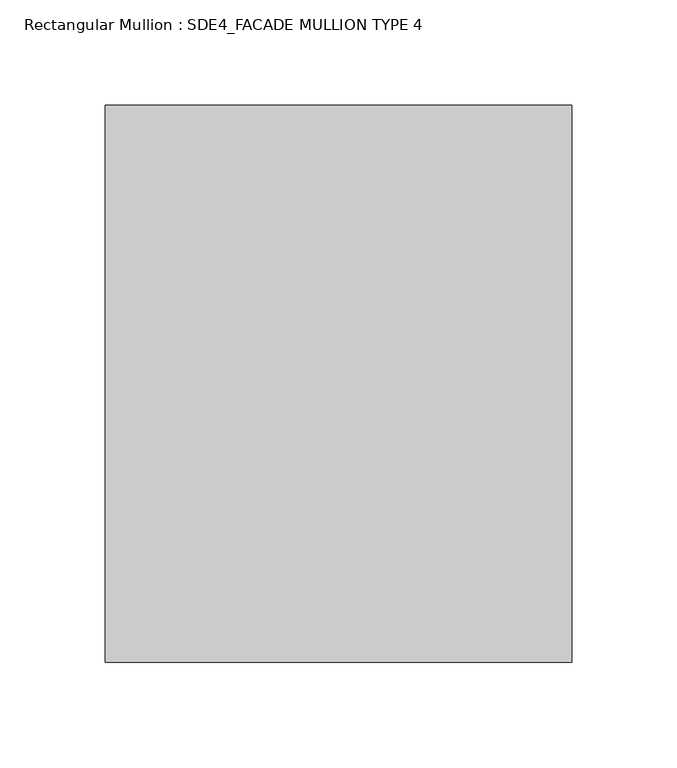
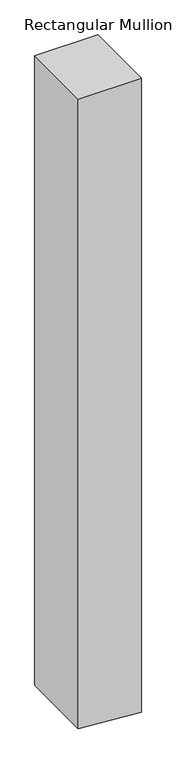
"""IFC4 building model written with IfcOpenShell, lengths in millimetres: member geometry, Rectangular Mullion : SDE4_FACADE MULLION TYPE 4."""

import ifcopenshell
import ifcopenshell.guid

model = None  # the IFC model being written
_history = None  # IfcOwnerHistory: only IFC2X3 demands one
_inside = {}  # id of a spatial element -> (the spatial element, [elements in it])
_under = {}  # id of a project, library or spatial element -> (it, [spatial elements below it])
_declared = {}  # id of a project -> (the project, [libraries it declares])
_typed = {}  # id of a type object -> (the type object, [elements of that type])
_made_of = {}  # id of a material, layer set ... -> (it, [elements and type objects made of it])


def new_model(schema):
    """Start an empty IFC model of exactly this schema.

    Asked for "IFC4X3", IfcOpenShell would pick the latest addendum, in which some entities
    have other attributes; the version numbers below select the first issue.
    IFC2X3 requires an IfcOwnerHistory on every rooted entity: one is made here for all.
    """
    global model, _history
    if schema == "IFC4X3":
        model = ifcopenshell.file(schema_version=(4, 3, 0, 0))
    else:
        model = ifcopenshell.file(schema=schema)
    _inside.clear()
    _under.clear()
    _declared.clear()
    _typed.clear()
    _made_of.clear()
    _history = None
    if model.schema == "IFC2X3":
        org = make("IfcOrganization", Name="unknown")
        user = make(
            "IfcPersonAndOrganization",
            ThePerson=make("IfcPerson", FamilyName="unknown"),
            TheOrganization=org,
        )
        app = make(
            "IfcApplication",
            ApplicationDeveloper=org,
            Version="unknown",
            ApplicationFullName="unknown",
            ApplicationIdentifier="unknown",
        )
        _history = make(
            "IfcOwnerHistory",
            OwningUser=user,
            OwningApplication=app,
            ChangeAction="ADDED",
            CreationDate=0,
        )
    return model


def make(cls, **values):
    """One entity of the class cls with the attributes given. An attribute that is None is left unset."""
    return model.create_entity(
        cls, **{name: value for name, value in values.items() if value is not None}
    )


def rooted(cls, **values):
    """An entity with a GlobalId (a new one), such as an element, a storey or a relation."""
    return make(cls, GlobalId=ifcopenshell.guid.new(), OwnerHistory=_history, **values)


def si_unit(unit_type, name, prefix=None):
    """IfcSIUnit, for example si_unit("LENGTHUNIT", "METRE", prefix="MILLI")."""
    return make("IfcSIUnit", UnitType=unit_type, Prefix=prefix, Name=name)


def assignment(units):
    """IfcUnitAssignment: the units of a project."""
    return None if units is None else make("IfcUnitAssignment", Units=units)


def point(xyz):
    """IfcCartesianPoint."""
    return None if xyz is None else make("IfcCartesianPoint", Coordinates=xyz)


def direction(xyz):
    """IfcDirection."""
    return None if xyz is None else make("IfcDirection", DirectionRatios=xyz)


def frame(location, z_axis=None, x_axis=None):
    """IfcAxis2Placement3D, a coordinate frame: its origin and axes. An axis left out is left unset."""
    return make(
        "IfcAxis2Placement3D",
        Location=point(location),
        Axis=direction(z_axis),
        RefDirection=direction(x_axis),
    )


def origin():
    """The frame at (0, 0, 0) with its axes left unset."""
    return frame((0.0, 0.0, 0.0))


def place(relative_to, where):
    """IfcLocalPlacement: puts the frame where relative to a parent placement (None: the world)."""
    return make(
        "IfcLocalPlacement", PlacementRelTo=relative_to, RelativePlacement=where
    )


def context(
    kind, dimensions, precision=None, world=None, true_north=None, identifier=None
):
    """IfcGeometricRepresentationContext, for example the 3D "Model" context."""
    return make(
        "IfcGeometricRepresentationContext",
        ContextIdentifier=identifier,
        ContextType=kind,
        CoordinateSpaceDimension=dimensions,
        Precision=precision,
        WorldCoordinateSystem=world,
        TrueNorth=true_north,
    )


def project(units=None, contexts=None):
    """IfcProject with its units and contexts."""
    return rooted(
        "IfcProject",
        Name="project",
        RepresentationContexts=contexts,
        UnitsInContext=assignment(units),
    )


def spatial(cls, under=None, at=None, **own):
    """A site, building, storey or space (cls), placed at a placement, below another one or the project."""
    s = rooted(cls, ObjectPlacement=at, **own)
    if under is not None:
        _under.setdefault(under.id(), (under, []))[1].append(s)
    return s


def polyline(points):
    """IfcPolyline through the points."""
    return make("IfcPolyline", Points=[point(p) for p in points])


def outline(outer, holes=None, kind="AREA"):
    """IfcArbitraryClosedProfileDef: a profile drawn as a closed curve; with holes, ...WithVoids."""
    if holes is None:
        return make("IfcArbitraryClosedProfileDef", ProfileType=kind, OuterCurve=outer)
    return make(
        "IfcArbitraryProfileDefWithVoids",
        ProfileType=kind,
        OuterCurve=outer,
        InnerCurves=holes,
    )


def extrude(swept, where, along, depth):
    """IfcExtrudedAreaSolid: the profile swept, set in the frame where, extruded along a direction by depth."""
    return make(
        "IfcExtrudedAreaSolid",
        SweptArea=swept,
        Position=where,
        ExtrudedDirection=direction(along),
        Depth=depth,
    )


def shape(context_of_items, identifier, shape_type, items):
    """IfcShapeRepresentation: the items that make up one representation, for example the "Body"."""
    return make(
        "IfcShapeRepresentation",
        ContextOfItems=context_of_items,
        RepresentationIdentifier=identifier,
        RepresentationType=shape_type,
        Items=items,
    )


def source(mapping_origin, context_of_items, identifier, shape_type, items):
    """IfcRepresentationMap: a shape defined once, which mapped items show again and again."""
    return make(
        "IfcRepresentationMap",
        MappingOrigin=mapping_origin,
        MappedRepresentation=shape(context_of_items, identifier, shape_type, items),
    )


def transform(
    local_origin,
    x_axis=None,
    y_axis=None,
    z_axis=None,
    scale=None,
    scale2=None,
    scale3=None,
    uniform=True,
):
    """IfcCartesianTransformationOperator3D, or its non-uniform kind. x_axis, y_axis, z_axis: its Axis1, 2, 3."""
    if uniform:
        return make(
            "IfcCartesianTransformationOperator3D",
            Axis1=direction(x_axis),
            Axis2=direction(y_axis),
            LocalOrigin=point(local_origin),
            Scale=scale,
            Axis3=direction(z_axis),
        )
    return make(
        "IfcCartesianTransformationOperator3DnonUniform",
        Axis1=direction(x_axis),
        Axis2=direction(y_axis),
        LocalOrigin=point(local_origin),
        Scale=scale,
        Axis3=direction(z_axis),
        Scale2=scale2,
        Scale3=scale3,
    )


def mapped(mapping_source, mapping_target):
    """IfcMappedItem: shows the shape of a source again, moved by a transform."""
    return make(
        "IfcMappedItem", MappingSource=mapping_source, MappingTarget=mapping_target
    )


def made_of(thing, what):
    """Note that an element or type object is made of a material, layer set ...; save() writes the relation."""
    if what is not None:
        _made_of.setdefault(what.id(), (what, []))[1].append(thing)
    return thing


def element(
    cls,
    number,
    at=None,
    inside=None,
    cuts=None,
    type_object=None,
    material=None,
    context=None,
    identifier="Body",
    shape_type=None,
    held_by="IfcProductDefinitionShape",
    body=None,
    shapes=None,
    **own,
):
    """One element of the class cls, such as IfcWall. Its Tag is "e" and its number.

    at: its placement. inside: the storey or other place that contains it. cuts: it is an
    opening in that element (IfcRelVoidsElement). A single representation is given by context,
    identifier, shape_type and body (its items); several are given by shapes. held_by: the class
    of the entity that holds the representations. save() writes the other relations.
    """
    e = rooted(cls, Tag="e%d" % number, ObjectPlacement=at, **own)
    if body is not None:
        shapes = [shape(context, identifier, shape_type, body)]
    if shapes is not None:
        e.Representation = make(held_by, Representations=shapes)
    if inside is not None:
        _inside.setdefault(inside.id(), (inside, []))[1].append(e)
    if cuts is not None:
        rooted(
            "IfcRelVoidsElement", RelatingBuildingElement=cuts, RelatedOpeningElement=e
        )
    if type_object is not None:
        _typed.setdefault(type_object.id(), (type_object, []))[1].append(e)
    return made_of(e, material)


def aggregate(whole, parts):
    """IfcRelAggregates: a whole, such as a stair, and the parts it consists of."""
    return rooted("IfcRelAggregates", RelatingObject=whole, RelatedObjects=parts)


def save(model, path):
    """Write the relations noted so far, then the file.

    IfcRelAggregates (storeys below a building ...), IfcRelContainedInSpatialStructure (elements
    in a storey), IfcRelDefinesByType, IfcRelAssociatesMaterial and IfcRelDeclares: one each for
    every whole, place, type object, material and project.
    """
    for whole, parts in _under.values():
        aggregate(whole, parts)
    for where, things in _inside.values():
        rooted(
            "IfcRelContainedInSpatialStructure",
            RelatedElements=things,
            RelatingStructure=where,
        )
    for kind, things in _typed.values():
        rooted("IfcRelDefinesByType", RelatedObjects=things, RelatingType=kind)
    for what, things in _made_of.values():
        rooted("IfcRelAssociatesMaterial", RelatedObjects=things, RelatingMaterial=what)
    for by, libraries in _declared.values():
        rooted("IfcRelDeclares", RelatingContext=by, RelatedDefinitions=libraries)
    model.write(path)


def rectangular_mullion_sde4_facade_mullion_type_4_b9bd4984(model_context):
    return source(origin(), model_context, "Body", "SweptSolid", [
        extrude(outline(polyline([(0.0, 111.0), (0.0, -111.0), (-2340.7370328, -111.0), (-2349.4779545, 3.056508), (-2357.7503943, 111.0), (0.0, 111.0)])), frame((0.0, -132.5, 0.0), z_axis=(0.0, 1.0, 0.0), x_axis=(0.0, 0.0, 1.0)), (0.0, 0.0, 1.0), 265.0),
    ])


if __name__ == "__main__":
    model = new_model("IFC4")
    model_context = context("Model", 3, world=origin())
    ifc_project = project(units=[si_unit("LENGTHUNIT", "METRE", prefix="MILLI")], contexts=[model_context])
    site = spatial("IfcSite", under=ifc_project)
    building = spatial("IfcBuilding", under=site)
    placement = place(None, origin())
    rectangular_mullion_sde4_facade_mullion_type_4_shape = rectangular_mullion_sde4_facade_mullion_type_4_b9bd4984(model_context)
    element("IfcMember", 1, ObjectType="Rectangular Mullion : SDE4_FACADE MULLION TYPE 4", at=placement, inside=building, context=model_context, shape_type="MappedRepresentation", body=[
        mapped(rectangular_mullion_sde4_facade_mullion_type_4_shape, transform((0.0, 0.0, 0.0), x_axis=(1.0, 0.0, 0.0), y_axis=(0.0, 1.0, 0.0), z_axis=(0.0, 0.0, 1.0))),
    ])
    save(model, "model.ifc")

# Revit data of these elements
# Type "Rectangular Mullion : SDE4_FACADE MULLION TYPE 4"
#   built-in parameter 1007322 = 0.869423 (stored number, unit not read)
#   built-in parameter 1007321 = 0.364173 (stored number, unit not read)
#   built-in parameter 1007320 = 0.364173 (stored number, unit not read)
